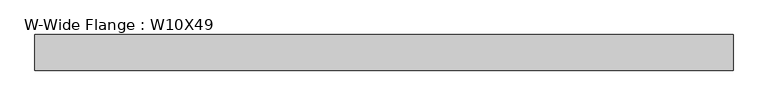
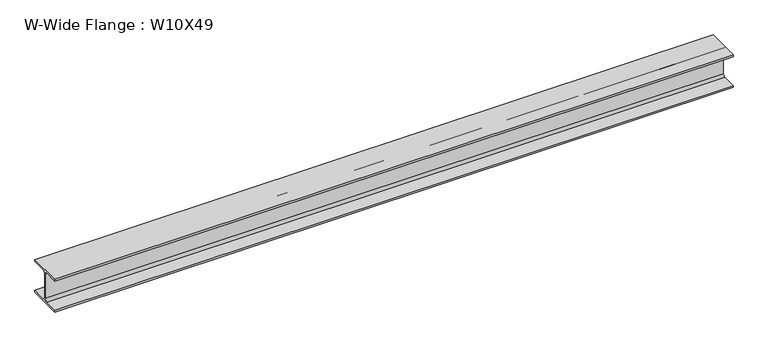
"""IFC4 building model written with IfcOpenShell, lengths in millimetres: beam geometry, W-Wide Flange : W10X49."""

from ifc_helpers import new_model, si_unit, point, frame, frame_2d, origin, place, context, project, spatial, polyline, circle_curve, trimmed, segment, composite_curve, outline, extrude, source, transform, mapped, element, save


def w_wide_flange_w10x49_791f69d4(model_context):
    return source(origin(), model_context, "Body", "SweptSolid", [
        extrude(outline(composite_curve([segment(polyline([(127.0, -112.776), (127.0, -127.0), (-127.0, -127.0), (-127.0, -112.776), (-21.844, -112.776)]), True, "CONTINUOUS"), segment(trimmed(circle_curve(frame_2d((-21.844, -95.25)), 17.526), [point((-21.844, -112.776))], [point((-4.318, -95.25))], True, "CARTESIAN"), True, "CONTINUOUS"), segment(polyline([(-4.318, -95.25), (-4.318, 95.25)]), True, "CONTINUOUS"), segment(trimmed(circle_curve(frame_2d((-21.844, 95.25)), 17.526), [point((-4.318, 95.25))], [point((-21.844, 112.776))], True, "CARTESIAN"), True, "CONTINUOUS"), segment(polyline([(-21.844, 112.776), (-127.0, 112.776), (-127.0, 127.0), (127.0, 127.0), (127.0, 112.776), (21.844, 112.776)]), True, "CONTINUOUS"), segment(trimmed(circle_curve(frame_2d((21.844, 95.25)), 17.526), [point((21.844, 112.776))], [point((4.318, 95.25))], True, "CARTESIAN"), True, "CONTINUOUS"), segment(polyline([(4.318, 95.25), (4.318, -95.25)]), True, "CONTINUOUS"), segment(trimmed(circle_curve(frame_2d((21.844, -95.25)), 17.526), [point((4.318, -95.25))], [point((21.844, -112.776))], True, "CARTESIAN"), True, "CONTINUOUS"), segment(polyline([(21.844, -112.776), (127.0, -112.776)]), True, "CONTINUOUS")], self_intersect=False)), frame((-2513.2454008, 0.0, 0.0), z_axis=(1.0, 0.0, 0.0), x_axis=(0.0, 1.0, 0.0)), (0.0, 0.0, 1.0), 4979.8450706),
    ])


if __name__ == "__main__":
    model = new_model("IFC4")
    model_context = context("Model", 3, world=origin())
    ifc_project = project(units=[si_unit("LENGTHUNIT", "METRE", prefix="MILLI")], contexts=[model_context])
    site = spatial("IfcSite", under=ifc_project)
    building = spatial("IfcBuilding", under=site)
    placement = place(None, origin())
    w_wide_flange_w10x49_shape = w_wide_flange_w10x49_791f69d4(model_context)
    element("IfcBeam", 1, ObjectType="W-Wide Flange : W10X49", at=placement, inside=building, context=model_context, shape_type="MappedRepresentation", body=[
        mapped(w_wide_flange_w10x49_shape, transform((0.0, 0.0, 0.0), x_axis=(1.0, 0.0, 0.0), y_axis=(0.0, 1.0, 0.0), z_axis=(0.0, 0.0, 1.0))),
    ])
    save(model, "model.ifc")

# Revit data of these elements
# Type "W-Wide Flange : W10X49"
#   Assembly Code = "B10"
#   W = 49
#   Length [instance default] = 1524 mm
#   bf = 254 mm
#   d = 254 mm
#   k = 31.75 mm
#   k2 = 17.526 mm
#   tf = 14.224 mm
#   tw = 8.636 mm
#   A = 0.0092903 m²
#   Structural Material [instance default] = Steel ASTM A992
# Element 1 (IfcBeam, "W-Wide Flange : W10X49")
#   Structural Material = Aluminum, Anodized Red
#   Materials on its faces: "Aluminum, Anodized Red"
# Materials
#   "Steel ASTM A992": class "Metal", colour RGB 128 0 0, transparency 0, Description = "Structural steel 50ksi", Cost = 0
#   "Aluminum, Anodized Red": class "Metal", colour RGB 120 120 120, transparency 0, Description = "Anodized aluminum, red", Cost = 0
